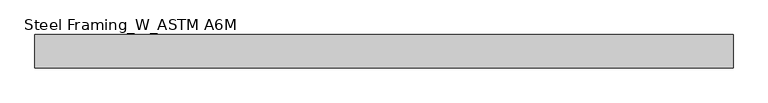
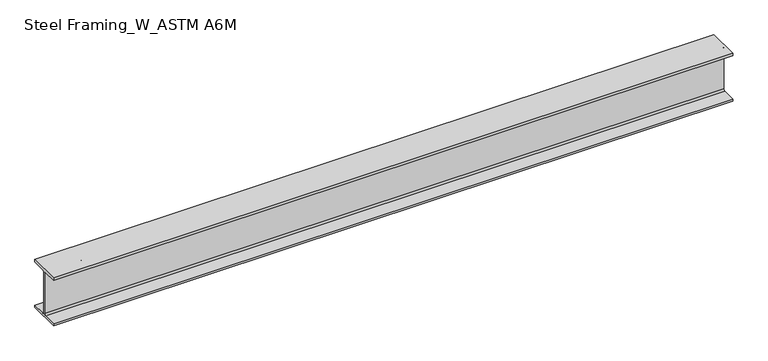
"""IFC4 building model written with IfcOpenShell, lengths in millimetres: beam geometry, Steel Framing_W_ASTM A6M : H_SB_AR_S02_W200x31.3_B6."""

from ifc_helpers import new_model, si_unit, point, frame, frame_2d, origin, place, context, project, spatial, polyline, circle_curve, trimmed, segment, composite_curve, outline, extrude, source, transform, mapped, element, save


def steel_framing_w_astm_a6m_8d3d16c6(model_context):
    return source(origin(), model_context, "Body", "SweptSolid", [
        extrude(outline(composite_curve([segment(polyline([(67.0, -94.8), (67.0, -105.0), (-67.0, -105.0), (-67.0, -94.8), (-10.775, -94.8)]), True, "CONTINUOUS"), segment(trimmed(circle_curve(frame_2d((-10.775, -87.2)), 7.6), [point((-10.775, -94.8))], [point((-3.175, -87.2))], True, "CARTESIAN"), True, "CONTINUOUS"), segment(polyline([(-3.175, -87.2), (-3.175, 87.2)]), True, "CONTINUOUS"), segment(trimmed(circle_curve(frame_2d((-10.775, 87.2)), 7.6), [point((-3.175, 87.2))], [point((-10.775, 94.8))], True, "CARTESIAN"), True, "CONTINUOUS"), segment(polyline([(-10.775, 94.8), (-67.0, 94.8), (-67.0, 105.0), (67.0, 105.0), (67.0, 94.8), (10.775, 94.8)]), True, "CONTINUOUS"), segment(trimmed(circle_curve(frame_2d((10.775, 87.2)), 7.6), [point((10.775, 94.8))], [point((3.175, 87.2))], True, "CARTESIAN"), True, "CONTINUOUS"), segment(polyline([(3.175, 87.2), (3.175, -87.2)]), True, "CONTINUOUS"), segment(trimmed(circle_curve(frame_2d((10.775, -87.2)), 7.6), [point((3.175, -87.2))], [point((10.775, -94.8))], True, "CARTESIAN"), True, "CONTINUOUS"), segment(polyline([(10.775, -94.8), (67.0, -94.8)]), True, "CONTINUOUS")], self_intersect=False)), frame((-1382.2, 0.0, 0.0), z_axis=(1.0, 0.0, 0.0), x_axis=(0.0, 1.0, 0.0)), (0.0, 0.0, 1.0), 2813.1),
    ])


if __name__ == "__main__":
    model = new_model("IFC4")
    model_context = context("Model", 3, world=origin())
    ifc_project = project(units=[si_unit("LENGTHUNIT", "METRE", prefix="MILLI")], contexts=[model_context])
    site = spatial("IfcSite", under=ifc_project)
    building = spatial("IfcBuilding", under=site)
    placement = place(None, origin())
    steel_framing_w_astm_a6m_shape = steel_framing_w_astm_a6m_8d3d16c6(model_context)
    element("IfcBeam", 1, ObjectType="Steel Framing_W_ASTM A6M : H_SB_AR_S02_W200x31.3_B6", at=placement, inside=building, context=model_context, shape_type="MappedRepresentation", body=[
        mapped(steel_framing_w_astm_a6m_shape, transform((0.0, 0.0, 0.0), x_axis=(1.0, 0.0, 0.0), y_axis=(0.0, 1.0, 0.0), z_axis=(0.0, 0.0, 1.0))),
    ])
    save(model, "model.ifc")

# Revit data of these elements
# Type "Steel Framing_W_ASTM A6M : H_SB_AR_S02_W200x31.3_B6"
#   Type Mark = "B6"
#   Section Name Key = "W8x21"
#   Width = 13.4 cm
#   Web Thickness = 0.635 cm
#   Web Fillet = 0.76 cm
#   Warping Constant = 40800.0 cm⁶
#   Torsional Moment of Inertia = 11.70 cm⁴
#   Section Area = 39.7 cm²
#   Plastic Modulus weak axis = 93.2 cm³
#   Plastic Modulus strong axis = 334.0 cm³
#   Perimeter = 0.93 m²/m
#   Nominal Weight = 31.30 kgf/m
#   Moment of Inertia weak axis = 407.00 cm⁴
#   Moment of Inertia strong axis = 3130.00 cm⁴
#   Height = 21.0 cm
#   Flange Thickness = 1.02 cm
#   Elastic Modulus weak axis = 60.8 cm³
#   Elastic Modulus strong axis = 298.0 cm³
#   Centroid Vertical = 10.5 cm
#   Centroid Horizontal = 6.7 cm
#   Length [instance default] = 1500 mm
#   Structural Material [instance default] = Steel, 45-345
#   Bolt Spacing = 0
#   Assembly Code = ""
# Element 1 (IfcBeam, "Steel Framing_W_ASTM A6M : H_SB_AR_S02_W200x31.3_B6")
#   Materials on its faces: "Steel, 45-345"
# Materials
#   "Steel, 45-345": class "Metal", colour RGB 189 187 185, transparency 0, Description = "Steel 345 MPa", Cost = 0
